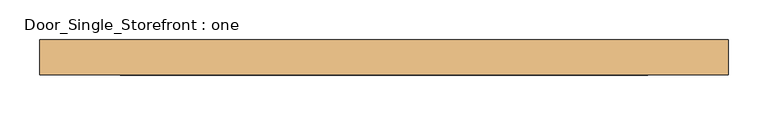
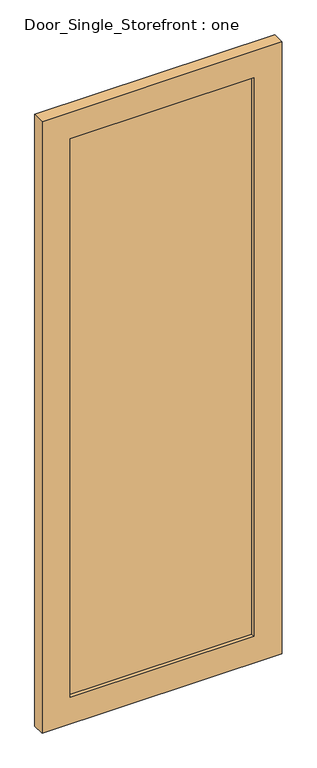
"""IFC4 building model written with IfcOpenShell, lengths in millimetres: door geometry, Door_Single_Storefront : one."""

from ifc_helpers import new_model, si_unit, frame, origin, place, context, project, spatial, polyline, outline, extrude, source, transform, mapped, element, save


def door_single_storefront_one_a4c326e9(model_context):
    return source(origin(), model_context, "Body", "SweptSolid", [
        extrude(outline(polyline([(2336.8, -434.18125), (0.0, -434.18125), (0.0, 434.18125), (2336.8, 434.18125), (2336.8, -434.18125)]), holes=[polyline([(101.6, 332.58125), (101.6, -332.58125), (2235.2, -332.58125), (2235.2, 332.58125), (101.6, 332.58125)])]), frame((0.0, 6.35, 0.0), z_axis=(0.0, 1.0, 0.0), x_axis=(0.0, 0.0, 1.0)), (0.0, 0.0, 1.0), 44.45),
        extrude(outline(polyline([(332.58125, 19.05), (-332.58125, 19.05), (-332.58125, 38.1), (332.58125, 38.1), (332.58125, 19.05)])), frame((0.0, 0.0, 101.6), z_axis=(0.0, 0.0, 1.0), x_axis=(1.0, 0.0, 0.0)), (0.0, 0.0, 1.0), 2133.6),
    ])


if __name__ == "__main__":
    model = new_model("IFC4")
    model_context = context("Model", 3, world=origin())
    ifc_project = project(units=[si_unit("LENGTHUNIT", "METRE", prefix="MILLI")], contexts=[model_context])
    site = spatial("IfcSite", under=ifc_project)
    building = spatial("IfcBuilding", under=site)
    placement = place(None, origin())
    door_single_storefront_one_shape = door_single_storefront_one_a4c326e9(model_context)
    element("IfcDoor", 1, ObjectType="Door_Single_Storefront : one", at=placement, inside=building, context=model_context, shape_type="MappedRepresentation", body=[
        mapped(door_single_storefront_one_shape, transform((0.0, 0.0, 0.0), x_axis=(1.0, 0.0, 0.0), y_axis=(0.0, 1.0, 0.0), z_axis=(0.0, 0.0, 1.0))),
    ])
    save(model, "model.ifc")

# Revit data of these elements
# Type "Door_Single_Storefront : one"
#   Type Mark = "27"
#   Analytic Construction = "<None>"
#   Stile_Width = 0' - 4"
#   Door_Thickness = 0' - 1 3/4"
#   Door_Offset = 0' - 2"
#   Glass_Material = Glass
#   Frame_Material = Aluminum
#   Function = (empty or 0)
# Element 1 (IfcDoor, "Door_Single_Storefront : one")
#   Materials on its faces: "Aluminum", "Glass"
# Materials
#   "Glass": class "Glass", colour RGB 0 128 192, transparency 0.75, Description = "Soda Lime Glass", Cost = 0
#   "Aluminum": class "Metal", colour RGB 247 247 247, transparency 0, Description = "Aluminum 6061", Cost = 0
